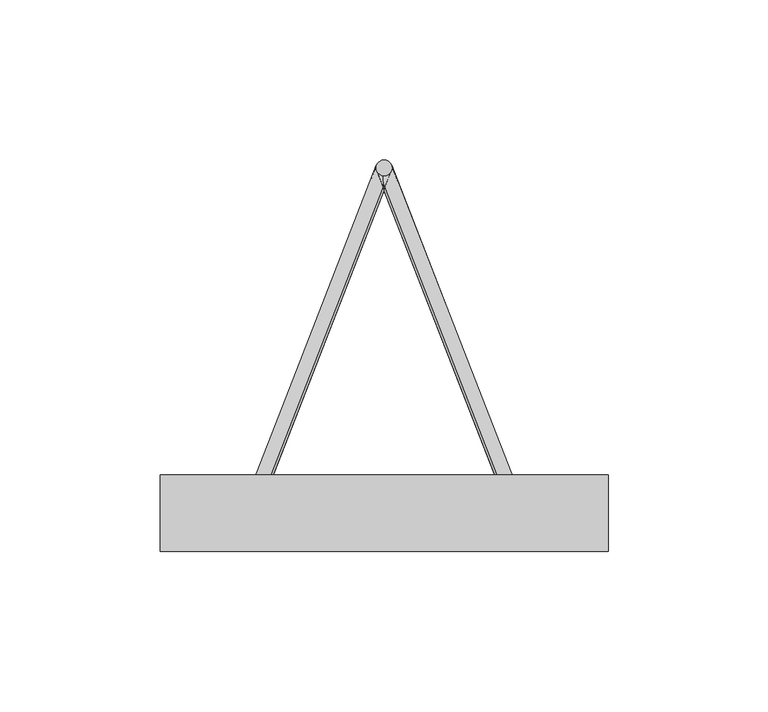
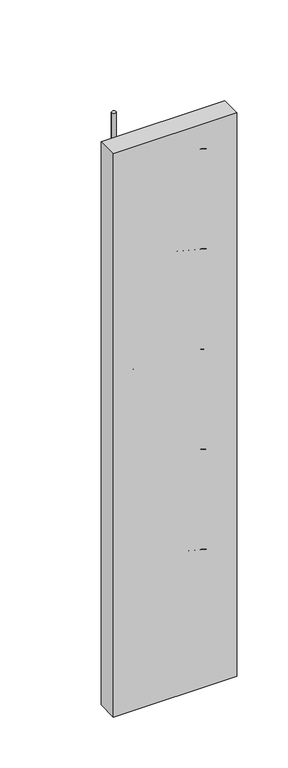
"""IFC4 building model written with IfcOpenShell, lengths in millimetres: proxy geometry, Vigota 1 (Pano 19) (Mf = 52)."""

from ifc_helpers import new_model, si_unit, point, frame, frame_2d, origin, origin_with_axes, origin_2d, place, context, project, spatial, polyline, circle_curve, trimmed, segment, composite_curve, outline, extrude, source, transform, mapped, element, save


def structural_framing_816a11a9(model_context):
    return source(origin(), model_context, "Body", "SweptSolid", [
        extrude(outline(polyline([(-70.0, 12.0), (70.0, 12.0), (70.0, -12.0), (-70.0, -12.0), (-70.0, 12.0)])), origin_with_axes(), (0.0, 0.0, 1.0), 675.0),
        extrude(outline(composite_curve([segment(trimmed(circle_curve(frame_2d((42.0, 0.0)), 2.5), [point((44.5, 0.0))], [point((39.5, 0.0))], False, "CARTESIAN"), True, "CONTINUOUS"), segment(trimmed(circle_curve(frame_2d((42.0, 0.0)), 2.5), [point((39.5, 0.0))], [point((44.5, 0.0))], False, "CARTESIAN"), True, "CONTINUOUS")], self_intersect=False)), frame((0.0, 0.0, 28.0), z_axis=(0.0, 0.0, 1.0), x_axis=(1.0, 0.0, 0.0)), (0.0, 0.0, 1.0), 619.0),
        extrude(outline(composite_curve([segment(trimmed(circle_curve(frame_2d((0.0, 108.0)), 2.5), [point((2.5, 108.0))], [point((-2.5, 108.0))], False, "CARTESIAN"), True, "CONTINUOUS"), segment(trimmed(circle_curve(frame_2d((0.0, 108.0)), 2.5), [point((-2.5, 108.0))], [point((2.5, 108.0))], False, "CARTESIAN"), True, "CONTINUOUS")], self_intersect=False)), frame((0.0, 0.0, 47.5), z_axis=(0.0, 0.0, 1.0), x_axis=(1.0, 0.0, 0.0)), (0.0, 0.0, 1.0), 580.0),
        extrude(outline(composite_curve([segment(trimmed(circle_curve(origin_2d(), 2.5), [point((2.5, 0.0))], [point((-2.5, 0.0))], False, "CARTESIAN"), True, "CONTINUOUS"), segment(trimmed(circle_curve(origin_2d(), 2.5), [point((-2.5, 0.0))], [point((2.5, 0.0))], False, "CARTESIAN"), True, "CONTINUOUS")], self_intersect=False)), frame((42.0, 0.0, 37.5), z_axis=(-0.3218603428886276, 0.8276408817707567, 0.4598004898837537), x_axis=(0.8192319205108605, -3.936835275445103e-11, 0.5734623443750141)), (0.0, 0.0, 1.0), 130.491379),
        extrude(outline(composite_curve([segment(trimmed(circle_curve(origin_2d(), 2.5), [point((2.5, 0.0))], [point((-2.5, 0.0))], False, "CARTESIAN"), True, "CONTINUOUS"), segment(trimmed(circle_curve(origin_2d(), 2.5), [point((-2.5, 0.0))], [point((2.5, 0.0))], False, "CARTESIAN"), True, "CONTINUOUS")], self_intersect=False)), frame((0.0, 108.0, 97.5), z_axis=(0.3218603428886276, -0.8276408817707567, 0.4598004898837537), x_axis=(0.8192319205108605, -3.936835275445103e-11, -0.5734623443750141)), (0.0, 0.0, 1.0), 130.491379),
        extrude(outline(composite_curve([segment(trimmed(circle_curve(origin_2d(), 2.5), [point((2.5, 0.0))], [point((-2.5, 0.0))], False, "CARTESIAN"), True, "CONTINUOUS"), segment(trimmed(circle_curve(origin_2d(), 2.5), [point((-2.5, 0.0))], [point((2.5, 0.0))], False, "CARTESIAN"), True, "CONTINUOUS")], self_intersect=False)), frame((42.0, 0.0, 157.5), z_axis=(-0.3218603428886276, 0.8276408817707567, 0.4598004898837537), x_axis=(0.8192319205108605, -3.936835275445103e-11, 0.5734623443750141)), (0.0, 0.0, 1.0), 130.491379),
        extrude(outline(composite_curve([segment(trimmed(circle_curve(origin_2d(), 2.5), [point((2.5, 0.0))], [point((-2.5, 0.0))], False, "CARTESIAN"), True, "CONTINUOUS"), segment(trimmed(circle_curve(origin_2d(), 2.5), [point((-2.5, 0.0))], [point((2.5, 0.0))], False, "CARTESIAN"), True, "CONTINUOUS")], self_intersect=False)), frame((0.0, 108.0, 217.5), z_axis=(0.3218603428886276, -0.8276408817707567, 0.4598004898837537), x_axis=(0.8192319205108605, -3.936835275445103e-11, -0.5734623443750141)), (0.0, 0.0, 1.0), 130.491379),
        extrude(outline(composite_curve([segment(trimmed(circle_curve(origin_2d(), 2.5), [point((2.5, 0.0))], [point((-2.5, 0.0))], False, "CARTESIAN"), True, "CONTINUOUS"), segment(trimmed(circle_curve(origin_2d(), 2.5), [point((-2.5, 0.0))], [point((2.5, 0.0))], False, "CARTESIAN"), True, "CONTINUOUS")], self_intersect=False)), frame((42.0, 0.0, 277.5), z_axis=(-0.3218603428886276, 0.8276408817707567, 0.4598004898837537), x_axis=(0.8192319205108605, -3.936835275445103e-11, 0.5734623443750141)), (0.0, 0.0, 1.0), 130.491379),
        extrude(outline(composite_curve([segment(trimmed(circle_curve(origin_2d(), 2.5), [point((2.5, 0.0))], [point((-2.5, 0.0))], False, "CARTESIAN"), True, "CONTINUOUS"), segment(trimmed(circle_curve(origin_2d(), 2.5), [point((-2.5, 0.0))], [point((2.5, 0.0))], False, "CARTESIAN"), True, "CONTINUOUS")], self_intersect=False)), frame((0.0, 108.0, 337.5), z_axis=(0.3218603428886276, -0.8276408817707567, 0.4598004898837537), x_axis=(0.8192319205108605, -3.936835275445103e-11, -0.5734623443750141)), (0.0, 0.0, 1.0), 130.491379),
        extrude(outline(composite_curve([segment(trimmed(circle_curve(origin_2d(), 2.5), [point((2.5, 0.0))], [point((-2.5, 0.0))], False, "CARTESIAN"), True, "CONTINUOUS"), segment(trimmed(circle_curve(origin_2d(), 2.5), [point((-2.5, 0.0))], [point((2.5, 0.0))], False, "CARTESIAN"), True, "CONTINUOUS")], self_intersect=False)), frame((42.0, 0.0, 397.5), z_axis=(-0.3218603428886276, 0.8276408817707567, 0.4598004898837537), x_axis=(0.8192319205108605, -3.936835275445103e-11, 0.5734623443750141)), (0.0, 0.0, 1.0), 130.491379),
        extrude(outline(composite_curve([segment(trimmed(circle_curve(origin_2d(), 2.5), [point((2.5, 0.0))], [point((-2.5, 0.0))], False, "CARTESIAN"), True, "CONTINUOUS"), segment(trimmed(circle_curve(origin_2d(), 2.5), [point((-2.5, 0.0))], [point((2.5, 0.0))], False, "CARTESIAN"), True, "CONTINUOUS")], self_intersect=False)), frame((0.0, 108.0, 457.5), z_axis=(0.3218603428886276, -0.8276408817707567, 0.4598004898837537), x_axis=(0.8192319205108605, -3.936835275445103e-11, -0.5734623443750141)), (0.0, 0.0, 1.0), 130.491379),
        extrude(outline(composite_curve([segment(trimmed(circle_curve(origin_2d(), 2.5), [point((2.5, 0.0))], [point((-2.5, 0.0))], False, "CARTESIAN"), True, "CONTINUOUS"), segment(trimmed(circle_curve(origin_2d(), 2.5), [point((-2.5, 0.0))], [point((2.5, 0.0))], False, "CARTESIAN"), True, "CONTINUOUS")], self_intersect=False)), frame((42.0, 0.0, 517.5), z_axis=(-0.3218603428886276, 0.8276408817707567, 0.4598004898837537), x_axis=(0.8192319205108605, -3.936835275445103e-11, 0.5734623443750141)), (0.0, 0.0, 1.0), 130.491379),
        extrude(outline(composite_curve([segment(trimmed(circle_curve(origin_2d(), 2.5), [point((2.5, 0.0))], [point((-2.5, 0.0))], False, "CARTESIAN"), True, "CONTINUOUS"), segment(trimmed(circle_curve(origin_2d(), 2.5), [point((-2.5, 0.0))], [point((2.5, 0.0))], False, "CARTESIAN"), True, "CONTINUOUS")], self_intersect=False)), frame((0.0, 108.0, 577.5), z_axis=(0.3218603428886276, -0.8276408817707567, 0.4598004898837537), x_axis=(0.8192319205108605, -3.936835275445103e-11, -0.5734623443750141)), (0.0, 0.0, 1.0), 130.491379),
        extrude(outline(composite_curve([segment(trimmed(circle_curve(frame_2d((-42.0, 0.0)), 2.5), [point((-39.5, 0.0))], [point((-44.5, 0.0))], False, "CARTESIAN"), True, "CONTINUOUS"), segment(trimmed(circle_curve(frame_2d((-42.0, 0.0)), 2.5), [point((-44.5, 0.0))], [point((-39.5, 0.0))], False, "CARTESIAN"), True, "CONTINUOUS")], self_intersect=False)), frame((0.0, 0.0, 28.0), z_axis=(0.0, 0.0, 1.0), x_axis=(1.0, 0.0, 0.0)), (0.0, 0.0, 1.0), 619.0),
        extrude(outline(composite_curve([segment(trimmed(circle_curve(origin_2d(), 2.5), [point((2.5, 0.0))], [point((-2.5, 0.0))], False, "CARTESIAN"), True, "CONTINUOUS"), segment(trimmed(circle_curve(origin_2d(), 2.5), [point((-2.5, 0.0))], [point((2.5, 0.0))], False, "CARTESIAN"), True, "CONTINUOUS")], self_intersect=False)), frame((-42.0, 0.0, 37.5), z_axis=(0.3218603428886276, 0.8276408817707567, 0.4598004898837537), x_axis=(0.8192319205108605, 3.936835275445103e-11, -0.5734623443750141)), (0.0, 0.0, 1.0), 130.491379),
        extrude(outline(composite_curve([segment(trimmed(circle_curve(origin_2d(), 2.5), [point((2.5, 0.0))], [point((-2.5, 0.0))], False, "CARTESIAN"), True, "CONTINUOUS"), segment(trimmed(circle_curve(origin_2d(), 2.5), [point((-2.5, 0.0))], [point((2.5, 0.0))], False, "CARTESIAN"), True, "CONTINUOUS")], self_intersect=False)), frame((0.0, 108.0, 97.5), z_axis=(-0.3218603428886276, -0.8276408817707567, 0.4598004898837537), x_axis=(0.8192319205108605, 3.936835275445103e-11, 0.5734623443750141)), (0.0, 0.0, 1.0), 130.491379),
        extrude(outline(composite_curve([segment(trimmed(circle_curve(origin_2d(), 2.5), [point((2.5, 0.0))], [point((-2.5, 0.0))], False, "CARTESIAN"), True, "CONTINUOUS"), segment(trimmed(circle_curve(origin_2d(), 2.5), [point((-2.5, 0.0))], [point((2.5, 0.0))], False, "CARTESIAN"), True, "CONTINUOUS")], self_intersect=False)), frame((-42.0, 0.0, 157.5), z_axis=(0.3218603428886276, 0.8276408817707567, 0.4598004898837537), x_axis=(0.8192319205108605, 3.936835275445103e-11, -0.5734623443750141)), (0.0, 0.0, 1.0), 130.491379),
        extrude(outline(composite_curve([segment(trimmed(circle_curve(origin_2d(), 2.5), [point((2.5, 0.0))], [point((-2.5, 0.0))], False, "CARTESIAN"), True, "CONTINUOUS"), segment(trimmed(circle_curve(origin_2d(), 2.5), [point((-2.5, 0.0))], [point((2.5, 0.0))], False, "CARTESIAN"), True, "CONTINUOUS")], self_intersect=False)), frame((0.0, 108.0, 217.5), z_axis=(-0.3218603428886276, -0.8276408817707567, 0.4598004898837537), x_axis=(0.8192319205108605, 3.936835275445103e-11, 0.5734623443750141)), (0.0, 0.0, 1.0), 130.491379),
        extrude(outline(composite_curve([segment(trimmed(circle_curve(origin_2d(), 2.5), [point((2.5, 0.0))], [point((-2.5, 0.0))], False, "CARTESIAN"), True, "CONTINUOUS"), segment(trimmed(circle_curve(origin_2d(), 2.5), [point((-2.5, 0.0))], [point((2.5, 0.0))], False, "CARTESIAN"), True, "CONTINUOUS")], self_intersect=False)), frame((-42.0, 0.0, 277.5), z_axis=(0.3218603428886276, 0.8276408817707567, 0.4598004898837537), x_axis=(0.8192319205108605, 3.936835275445103e-11, -0.5734623443750141)), (0.0, 0.0, 1.0), 130.491379),
        extrude(outline(composite_curve([segment(trimmed(circle_curve(origin_2d(), 2.5), [point((2.5, 0.0))], [point((-2.5, 0.0))], False, "CARTESIAN"), True, "CONTINUOUS"), segment(trimmed(circle_curve(origin_2d(), 2.5), [point((-2.5, 0.0))], [point((2.5, 0.0))], False, "CARTESIAN"), True, "CONTINUOUS")], self_intersect=False)), frame((0.0, 108.0, 337.5), z_axis=(-0.3218603428886276, -0.8276408817707567, 0.4598004898837537), x_axis=(0.8192319205108605, 3.936835275445103e-11, 0.5734623443750141)), (0.0, 0.0, 1.0), 130.491379),
        extrude(outline(composite_curve([segment(trimmed(circle_curve(origin_2d(), 2.5), [point((2.5, 0.0))], [point((-2.5, 0.0))], False, "CARTESIAN"), True, "CONTINUOUS"), segment(trimmed(circle_curve(origin_2d(), 2.5), [point((-2.5, 0.0))], [point((2.5, 0.0))], False, "CARTESIAN"), True, "CONTINUOUS")], self_intersect=False)), frame((-42.0, 0.0, 397.5), z_axis=(0.3218603428886276, 0.8276408817707567, 0.4598004898837537), x_axis=(0.8192319205108605, 3.936835275445103e-11, -0.5734623443750141)), (0.0, 0.0, 1.0), 130.491379),
        extrude(outline(composite_curve([segment(trimmed(circle_curve(origin_2d(), 2.5), [point((2.5, 0.0))], [point((-2.5, 0.0))], False, "CARTESIAN"), True, "CONTINUOUS"), segment(trimmed(circle_curve(origin_2d(), 2.5), [point((-2.5, 0.0))], [point((2.5, 0.0))], False, "CARTESIAN"), True, "CONTINUOUS")], self_intersect=False)), frame((0.0, 108.0, 457.5), z_axis=(-0.3218603428886276, -0.8276408817707567, 0.4598004898837537), x_axis=(0.8192319205108605, 3.936835275445103e-11, 0.5734623443750141)), (0.0, 0.0, 1.0), 130.491379),
        extrude(outline(composite_curve([segment(trimmed(circle_curve(origin_2d(), 2.5), [point((2.5, 0.0))], [point((-2.5, 0.0))], False, "CARTESIAN"), True, "CONTINUOUS"), segment(trimmed(circle_curve(origin_2d(), 2.5), [point((-2.5, 0.0))], [point((2.5, 0.0))], False, "CARTESIAN"), True, "CONTINUOUS")], self_intersect=False)), frame((-42.0, 0.0, 517.5), z_axis=(0.3218603428886276, 0.8276408817707567, 0.4598004898837537), x_axis=(0.8192319205108605, 3.936835275445103e-11, -0.5734623443750141)), (0.0, 0.0, 1.0), 130.491379),
        extrude(outline(composite_curve([segment(trimmed(circle_curve(origin_2d(), 2.5), [point((2.5, 0.0))], [point((-2.5, 0.0))], False, "CARTESIAN"), True, "CONTINUOUS"), segment(trimmed(circle_curve(origin_2d(), 2.5), [point((-2.5, 0.0))], [point((2.5, 0.0))], False, "CARTESIAN"), True, "CONTINUOUS")], self_intersect=False)), frame((0.0, 108.0, 577.5), z_axis=(-0.3218603428886276, -0.8276408817707567, 0.4598004898837537), x_axis=(0.8192319205108605, 3.936835275445103e-11, 0.5734623443750141)), (0.0, 0.0, 1.0), 130.491379),
    ])


if __name__ == "__main__":
    model = new_model("IFC4")
    model_context = context("Model", 3, world=origin())
    ifc_project = project(units=[si_unit("LENGTHUNIT", "METRE", prefix="MILLI")], contexts=[model_context])
    site = spatial("IfcSite", under=ifc_project)
    building = spatial("IfcBuilding", under=site)
    placement = place(None, origin())
    structural_framing_shape = structural_framing_816a11a9(model_context)
    element("IfcBuildingElementProxy", 1, Name="Vigota 1 (Pano 19) (Mf = 52)", ObjectType="Vigota 1 (Pano 19) (Mf = 52)", at=placement, inside=building, context=model_context, shape_type="MappedRepresentation", body=[
        mapped(structural_framing_shape, transform((0.0, 0.0, 0.0), x_axis=(1.0, 0.0, 0.0), y_axis=(0.0, 1.0, 0.0), z_axis=(0.0, 0.0, 1.0))),
    ])
    save(model, "model.ifc")

# Revit data of these elements
# Element 1 (IfcBuildingElementProxy, "Vigota 1 (Pano 19) (Mf = 52)")
#   Materials on its faces: "Aço", "Concreto armado"
# Materials
#   "Aço": class "Metal", colour RGB 120 120 120, transparency 0, Description = "Aço estrutural A36 grau, ASTM B, acabamento laminado", Cost = 0
#   "Concreto armado": class "Não atribuído", colour RGB 168 169 158, transparency 0
